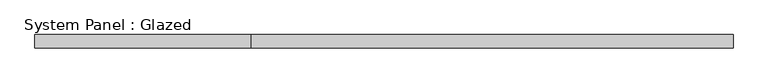
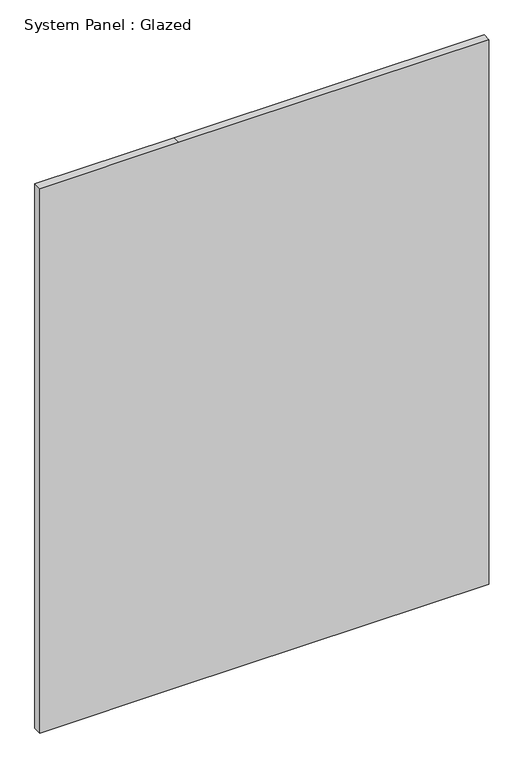
"""IFC4 building model written with IfcOpenShell, lengths in millimetres: plate geometry, System Panel : Glazed."""

from ifc_helpers import new_model, si_unit, frame, origin, place, context, project, spatial, polyline, outline, extrude, source, transform, mapped, element, save


def system_panel_glazed_1c059595(model_context):
    return source(origin(), model_context, "Body", "SweptSolid", [
        extrude(outline(polyline([(0.0, -676.275), (0.0, -257.175), (0.0, 676.275), (1733.55, 676.275), (1733.55, -257.175), (1733.55, -676.275), (0.0, -676.275)])), frame((0.0, -44.45, 0.0), z_axis=(0.0, 1.0, 0.0), x_axis=(0.0, 0.0, 1.0)), (0.0, 0.0, 1.0), 25.4),
    ])


if __name__ == "__main__":
    model = new_model("IFC4")
    model_context = context("Model", 3, world=origin())
    ifc_project = project(units=[si_unit("LENGTHUNIT", "METRE", prefix="MILLI")], contexts=[model_context])
    site = spatial("IfcSite", under=ifc_project)
    building = spatial("IfcBuilding", under=site)
    placement = place(None, origin())
    system_panel_glazed_shape = system_panel_glazed_1c059595(model_context)
    element("IfcPlate", 1, ObjectType="System Panel : Glazed", at=placement, inside=building, context=model_context, shape_type="MappedRepresentation", body=[
        mapped(system_panel_glazed_shape, transform((0.0, 0.0, 0.0), x_axis=(1.0, 0.0, 0.0), y_axis=(0.0, 1.0, 0.0), z_axis=(0.0, 0.0, 1.0))),
    ])
    save(model, "model.ifc")

# Revit data of these elements
# Type "System Panel : Glazed"
#   Construction Type Id = "GSP4R"
#   Analytic Construction = "1/8 in Pilkington single glazing"
#   Visual Light Transmittance = 0.9
#   Solar Heat Gain Coefficient = 0.86
#   Heat Transfer Coefficient (U) = 1.18115 BTU/(h·ft²·°F)
#   Define Thermal Properties by = 1
# Element 1 (IfcPlate, "System Panel : Glazed")
#   Materials on its faces: "Glass"
# Materials
#   "Glass": class "Glass", colour RGB 0 0 255, transparency 0.75, Description = "Soda Lime Glass", Cost = 0
